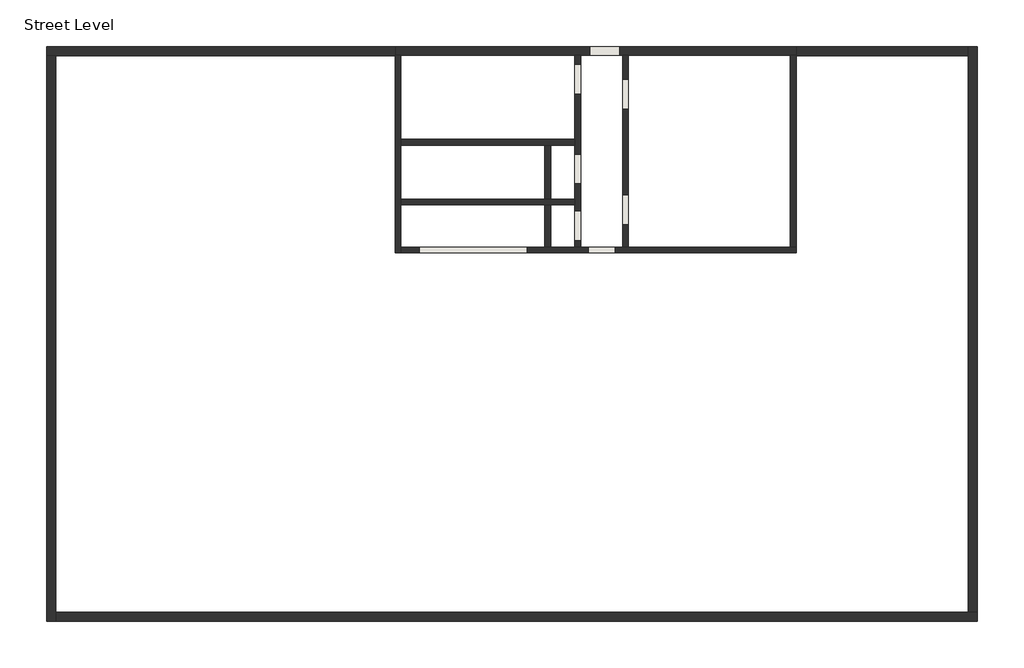
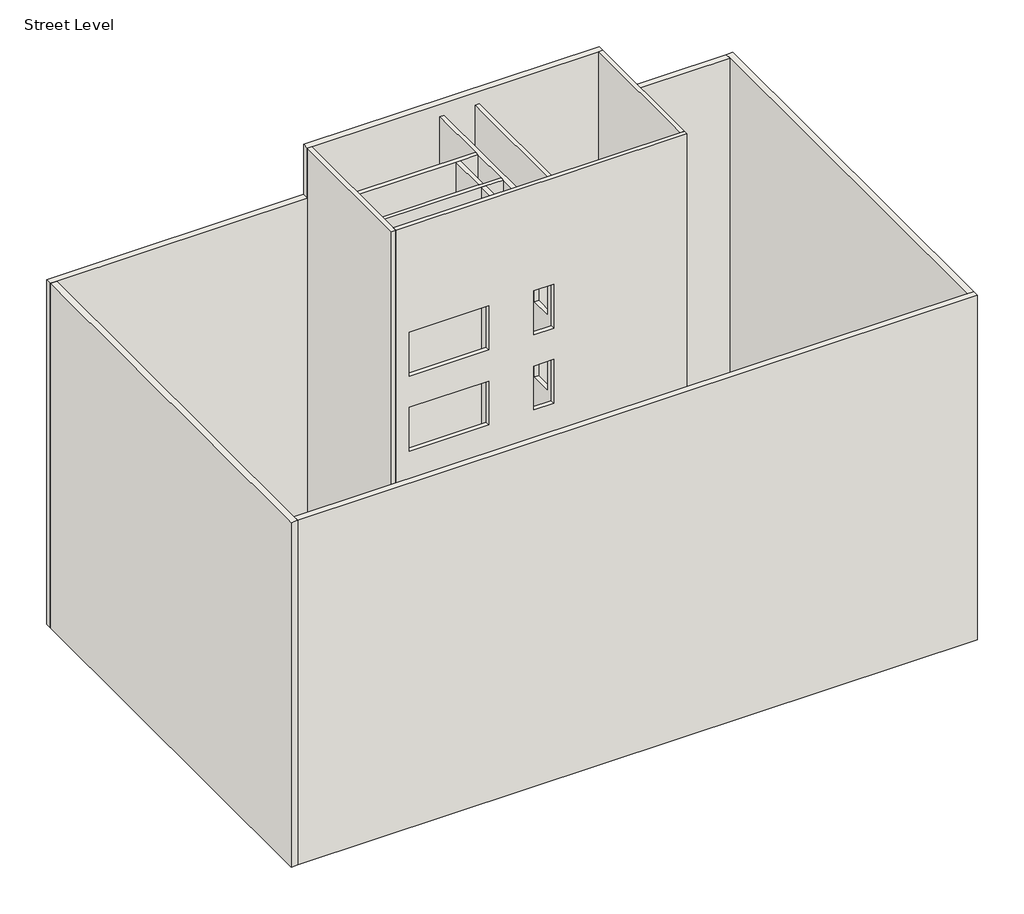
# One storey: 14 walls.
"""IFC4 building model written with IfcOpenShell, lengths in millimetres."""

import ifcopenshell
import ifcopenshell.guid

model = None  # the IFC model being written
_history = None  # IfcOwnerHistory: only IFC2X3 demands one
_inside = {}  # id of a spatial element -> (the spatial element, [elements in it])
_under = {}  # id of a project, library or spatial element -> (it, [spatial elements below it])
_declared = {}  # id of a project -> (the project, [libraries it declares])
_typed = {}  # id of a type object -> (the type object, [elements of that type])
_made_of = {}  # id of a material, layer set ... -> (it, [elements and type objects made of it])


def new_model(schema):
    """Start an empty IFC model of exactly this schema.

    Asked for "IFC4X3", IfcOpenShell would pick the latest addendum, in which some entities
    have other attributes; the version numbers below select the first issue.
    IFC2X3 requires an IfcOwnerHistory on every rooted entity: one is made here for all.
    """
    global model, _history
    if schema == "IFC4X3":
        model = ifcopenshell.file(schema_version=(4, 3, 0, 0))
    else:
        model = ifcopenshell.file(schema=schema)
    _inside.clear()
    _under.clear()
    _declared.clear()
    _typed.clear()
    _made_of.clear()
    _history = None
    if model.schema == "IFC2X3":
        org = make("IfcOrganization", Name="unknown")
        user = make(
            "IfcPersonAndOrganization",
            ThePerson=make("IfcPerson", FamilyName="unknown"),
            TheOrganization=org,
        )
        app = make(
            "IfcApplication",
            ApplicationDeveloper=org,
            Version="unknown",
            ApplicationFullName="unknown",
            ApplicationIdentifier="unknown",
        )
        _history = make(
            "IfcOwnerHistory",
            OwningUser=user,
            OwningApplication=app,
            ChangeAction="ADDED",
            CreationDate=0,
        )
    return model


def make(cls, **values):
    """One entity of the class cls with the attributes given. An attribute that is None is left unset."""
    return model.create_entity(
        cls, **{name: value for name, value in values.items() if value is not None}
    )


def rooted(cls, **values):
    """An entity with a GlobalId (a new one), such as an element, a storey or a relation."""
    return make(cls, GlobalId=ifcopenshell.guid.new(), OwnerHistory=_history, **values)


def si_unit(unit_type, name, prefix=None):
    """IfcSIUnit, for example si_unit("LENGTHUNIT", "METRE", prefix="MILLI")."""
    return make("IfcSIUnit", UnitType=unit_type, Prefix=prefix, Name=name)


def assignment(units):
    """IfcUnitAssignment: the units of a project."""
    return None if units is None else make("IfcUnitAssignment", Units=units)


def point(xyz):
    """IfcCartesianPoint."""
    return None if xyz is None else make("IfcCartesianPoint", Coordinates=xyz)


def direction(xyz):
    """IfcDirection."""
    return None if xyz is None else make("IfcDirection", DirectionRatios=xyz)


def frame(location, z_axis=None, x_axis=None):
    """IfcAxis2Placement3D, a coordinate frame: its origin and axes. An axis left out is left unset."""
    return make(
        "IfcAxis2Placement3D",
        Location=point(location),
        Axis=direction(z_axis),
        RefDirection=direction(x_axis),
    )


def origin():
    """The frame at (0, 0, 0) with its axes left unset."""
    return frame((0.0, 0.0, 0.0))


def place(relative_to, where):
    """IfcLocalPlacement: puts the frame where relative to a parent placement (None: the world)."""
    return make(
        "IfcLocalPlacement", PlacementRelTo=relative_to, RelativePlacement=where
    )


def context(
    kind, dimensions, precision=None, world=None, true_north=None, identifier=None
):
    """IfcGeometricRepresentationContext, for example the 3D "Model" context."""
    return make(
        "IfcGeometricRepresentationContext",
        ContextIdentifier=identifier,
        ContextType=kind,
        CoordinateSpaceDimension=dimensions,
        Precision=precision,
        WorldCoordinateSystem=world,
        TrueNorth=true_north,
    )


def project(units=None, contexts=None):
    """IfcProject with its units and contexts."""
    return rooted(
        "IfcProject",
        Name="project",
        RepresentationContexts=contexts,
        UnitsInContext=assignment(units),
    )


def spatial(cls, under=None, at=None, **own):
    """A site, building, storey or space (cls), placed at a placement, below another one or the project."""
    s = rooted(cls, ObjectPlacement=at, **own)
    if under is not None:
        _under.setdefault(under.id(), (under, []))[1].append(s)
    return s


def polyline(points):
    """IfcPolyline through the points."""
    return make("IfcPolyline", Points=[point(p) for p in points])


def outline(outer, holes=None, kind="AREA"):
    """IfcArbitraryClosedProfileDef: a profile drawn as a closed curve; with holes, ...WithVoids."""
    if holes is None:
        return make("IfcArbitraryClosedProfileDef", ProfileType=kind, OuterCurve=outer)
    return make(
        "IfcArbitraryProfileDefWithVoids",
        ProfileType=kind,
        OuterCurve=outer,
        InnerCurves=holes,
    )


def extrude(swept, where, along, depth):
    """IfcExtrudedAreaSolid: the profile swept, set in the frame where, extruded along a direction by depth."""
    return make(
        "IfcExtrudedAreaSolid",
        SweptArea=swept,
        Position=where,
        ExtrudedDirection=direction(along),
        Depth=depth,
    )


def faces_of(points, faces, orient=None, outer=None):
    """IfcFace entities. A face is a list of loops; a loop is a list of indices into points, from 0.

    orient and outer hold one flag for each loop. By default every Orientation is true, the
    first loop of a face is its IfcFaceOuterBound and the others are IfcFaceBound.
    """
    made = []
    for i, loops in enumerate(faces):
        bounds = []
        for j, loop in enumerate(loops):
            is_outer = j == 0 if outer is None else outer[i][j]
            bounds.append(
                make(
                    "IfcFaceOuterBound" if is_outer else "IfcFaceBound",
                    Bound=make("IfcPolyLoop", Polygon=[points[k] for k in loop]),
                    Orientation=True if orient is None else orient[i][j],
                )
            )
        made.append(make("IfcFace", Bounds=bounds))
    return made


def faceted_brep(points, faces, orient=None, outer=None, voids=None):
    """IfcFacetedBrep: a solid bounded by flat faces; with voids (closed shells), ...WithVoids."""
    shared = [point(p) for p in points]
    hull = make("IfcClosedShell", CfsFaces=faces_of(shared, faces, orient, outer))
    if voids is None:
        return make("IfcFacetedBrep", Outer=hull)
    return make(
        "IfcFacetedBrepWithVoids",
        Outer=hull,
        Voids=[
            make(cls, CfsFaces=faces_of(shared, fs, o, b)) for cls, fs, o, b in voids
        ],
    )


def shape(context_of_items, identifier, shape_type, items):
    """IfcShapeRepresentation: the items that make up one representation, for example the "Body"."""
    return make(
        "IfcShapeRepresentation",
        ContextOfItems=context_of_items,
        RepresentationIdentifier=identifier,
        RepresentationType=shape_type,
        Items=items,
    )


def made_of(thing, what):
    """Note that an element or type object is made of a material, layer set ...; save() writes the relation."""
    if what is not None:
        _made_of.setdefault(what.id(), (what, []))[1].append(thing)
    return thing


def element(
    cls,
    number,
    at=None,
    inside=None,
    cuts=None,
    type_object=None,
    material=None,
    context=None,
    identifier="Body",
    shape_type=None,
    held_by="IfcProductDefinitionShape",
    body=None,
    shapes=None,
    **own,
):
    """One element of the class cls, such as IfcWall. Its Tag is "e" and its number.

    at: its placement. inside: the storey or other place that contains it. cuts: it is an
    opening in that element (IfcRelVoidsElement). A single representation is given by context,
    identifier, shape_type and body (its items); several are given by shapes. held_by: the class
    of the entity that holds the representations. save() writes the other relations.
    """
    e = rooted(cls, Tag="e%d" % number, ObjectPlacement=at, **own)
    if body is not None:
        shapes = [shape(context, identifier, shape_type, body)]
    if shapes is not None:
        e.Representation = make(held_by, Representations=shapes)
    if inside is not None:
        _inside.setdefault(inside.id(), (inside, []))[1].append(e)
    if cuts is not None:
        rooted(
            "IfcRelVoidsElement", RelatingBuildingElement=cuts, RelatedOpeningElement=e
        )
    if type_object is not None:
        _typed.setdefault(type_object.id(), (type_object, []))[1].append(e)
    return made_of(e, material)


def aggregate(whole, parts):
    """IfcRelAggregates: a whole, such as a stair, and the parts it consists of."""
    return rooted("IfcRelAggregates", RelatingObject=whole, RelatedObjects=parts)


def save(model, path):
    """Write the relations noted so far, then the file.

    IfcRelAggregates (storeys below a building ...), IfcRelContainedInSpatialStructure (elements
    in a storey), IfcRelDefinesByType, IfcRelAssociatesMaterial and IfcRelDeclares: one each for
    every whole, place, type object, material and project.
    """
    for whole, parts in _under.values():
        aggregate(whole, parts)
    for where, things in _inside.values():
        rooted(
            "IfcRelContainedInSpatialStructure",
            RelatedElements=things,
            RelatingStructure=where,
        )
    for kind, things in _typed.values():
        rooted("IfcRelDefinesByType", RelatedObjects=things, RelatingType=kind)
    for what, things in _made_of.values():
        rooted("IfcRelAssociatesMaterial", RelatedObjects=things, RelatingMaterial=what)
    for by, libraries in _declared.values():
        rooted("IfcRelDeclares", RelatingContext=by, RelatedDefinitions=libraries)
    model.write(path)


model = new_model("IFC4")

# Units and contexts
model_context = context("Model", 3, world=origin())
ifc_project = project(units=[si_unit("LENGTHUNIT", "METRE", prefix="MILLI")], contexts=[model_context])

# Site, building, storey
site = spatial("IfcSite", under=ifc_project)
building = spatial("IfcBuilding", under=site)
storey = spatial("IfcBuildingStorey", under=building, Name="Street Level", Elevation=-914.4)

# Walls
placement = place(None, origin())
element("IfcWall", 1, ObjectType="Generic - 12\"", at=placement, inside=storey, context=model_context, shape_type="Brep", body=[
    faceted_brep([(-16964.6122732, 9291.5015304, -914.4), (-16659.8122732, 9291.5015304, -914.4), (-5128.2122732, 9291.5015304, -914.4), (-5128.2122732, 9291.5015304, 0.0), (-5128.2122732, 9291.5015304, 3657.6), (-5128.2122732, 9291.5015304, 7315.2), (-5128.2122732, 9291.5015304, 10972.8), (-5128.2122732, 9291.5015304, 14630.4), (-5128.2122732, 9291.5015304, 15849.6), (-16659.8122732, 9291.5015304, 15849.6), (-16964.6122732, 9291.5015304, 15849.6), (-16964.6122732, 9596.3015304, -914.4), (-16964.6122732, 9596.3015304, 15849.6), (-5128.2122732, 9596.3015304, 15849.6), (-5128.2122732, 9596.3015304, -914.4)], [[[0, 1, 2, 3, 4, 5, 6, 7, 8, 9, 10]], [[11, 12, 13, 14]], [[2, 1, 0, 11, 14]], [[10, 9, 8, 13, 12]], [[0, 10, 12, 11]], [[8, 7, 6, 5, 4, 3, 2, 14, 13]]]),
])
element("IfcWall", 2, ObjectType="Generic - 12\"", at=placement, inside=storey, context=model_context, shape_type="Brep", body=[
    faceted_brep([(-16659.8122732, -9910.8984696, -914.4), (-16659.8122732, -9606.0984696, -914.4), (-16659.8122732, 9291.5015304, -914.4), (-16659.8122732, 9291.5015304, 0.0), (-16659.8122732, 9291.5015304, 3657.6), (-16659.8122732, 9291.5015304, 7010.4), (-16659.8122732, 9291.5015304, 7315.2), (-16659.8122732, 9291.5015304, 10972.8), (-16659.8122732, 9291.5015304, 14630.4), (-16659.8122732, 9291.5015304, 15849.6), (-16659.8122732, -9606.0984696, 15849.6), (-16659.8122732, -9910.8984696, 15849.6), (-16964.6122732, -9910.8984696, -914.4), (-16964.6122732, -9910.8984696, 15849.6), (-16964.6122732, 9291.5015304, 15849.6), (-16964.6122732, 9291.5015304, -914.4)], [[[0, 1, 2, 3, 4, 5, 6, 7, 8, 9, 10, 11]], [[12, 13, 14, 15]], [[2, 1, 0, 12, 15]], [[11, 10, 9, 14, 13]], [[0, 11, 13, 12]], [[9, 8, 7, 6, 5, 4, 3, 2, 15, 14]]]),
])
element("IfcWall", 3, ObjectType="Generic - 12\"", at=placement, inside=storey, context=model_context, shape_type="Brep", body=[
    faceted_brep([(14632.9877268, -9606.0984696, -914.4), (14328.1877268, -9606.0984696, -914.4), (-16659.8122732, -9606.0984696, -914.4), (-16659.8122732, -9606.0984696, 0.0), (-16659.8122732, -9606.0984696, 3657.6), (-16659.8122732, -9606.0984696, 7010.4), (-16659.8122732, -9606.0984696, 7315.2), (-16659.8122732, -9606.0984696, 10972.8), (-16659.8122732, -9606.0984696, 14630.4), (-16659.8122732, -9606.0984696, 15849.6), (14328.1877268, -9606.0984696, 15849.6), (14632.9877268, -9606.0984696, 15849.6), (14632.9877268, -9910.8984696, -914.4), (14632.9877268, -9910.8984696, 15849.6), (-16659.8122732, -9910.8984696, 15849.6), (-16659.8122732, -9910.8984696, -914.4)], [[[0, 1, 2, 3, 4, 5, 6, 7, 8, 9, 10, 11]], [[12, 13, 14, 15]], [[2, 1, 0, 12, 15]], [[11, 10, 9, 14, 13]], [[0, 11, 13, 12]], [[9, 8, 7, 6, 5, 4, 3, 2, 15, 14]]]),
])
element("IfcWall", 4, ObjectType="Generic - 12\"", at=placement, inside=storey, context=model_context, shape_type="Brep", body=[
    faceted_brep([(14328.1877268, 9596.3015304, -914.4), (14328.1877268, 9291.5015304, -914.4), (14328.1877268, -9606.0984696, -914.4), (14328.1877268, -9606.0984696, 0.0), (14328.1877268, -9606.0984696, 3657.6), (14328.1877268, -9606.0984696, 7010.4), (14328.1877268, -9606.0984696, 7315.2), (14328.1877268, -9606.0984696, 10972.8), (14328.1877268, -9606.0984696, 14630.4), (14328.1877268, -9606.0984696, 15849.6), (14328.1877268, 9291.5015304, 15849.6), (14328.1877268, 9596.3015304, 15849.6), (14632.9877268, 9596.3015304, -914.4), (14632.9877268, 9596.3015304, 15849.6), (14632.9877268, -9606.0984696, 15849.6), (14632.9877268, -9606.0984696, -914.4)], [[[0, 1, 2, 3, 4, 5, 6, 7, 8, 9, 10, 11]], [[12, 13, 14, 15]], [[2, 1, 0, 12, 15]], [[11, 10, 9, 14, 13]], [[0, 11, 13, 12]], [[9, 8, 7, 6, 5, 4, 3, 2, 15, 14]]]),
])
element("IfcWall", 5, ObjectType="Generic - 12\"", at=placement, inside=storey, context=model_context, shape_type="Brep", body=[
    faceted_brep([(8476.6627268, 9291.5015304, -914.4), (14328.1877268, 9291.5015304, -914.4), (14328.1877268, 9291.5015304, 0.0), (14328.1877268, 9291.5015304, 3352.8), (14328.1877268, 9291.5015304, 3657.6), (14328.1877268, 9291.5015304, 7010.4), (14328.1877268, 9291.5015304, 7315.2), (14328.1877268, 9291.5015304, 10668.0), (14328.1877268, 9291.5015304, 10972.8), (14328.1877268, 9291.5015304, 14630.4), (14328.1877268, 9291.5015304, 15849.6), (8476.6627268, 9291.5015304, 15849.6), (8476.6627268, 9596.3015304, -914.4), (8476.6627268, 9596.3015304, 15849.6), (14328.1877268, 9596.3015304, 15849.6), (14328.1877268, 9596.3015304, -914.4)], [[[0, 1, 2, 3, 4, 5, 6, 7, 8, 9, 10, 11]], [[12, 13, 14, 15]], [[1, 0, 12, 15]], [[11, 10, 14, 13]], [[10, 9, 8, 7, 6, 5, 4, 3, 2, 1, 15, 14]], [[0, 11, 13, 12]]]),
])
element("IfcWall", 6, ObjectType="Generic - 12\" Masonry", at=placement, inside=storey, context=model_context, shape_type="Brep", body=[
    faceted_brep([(-5128.2122732, 9301.0265304, 18288.0), (-5128.2122732, 9301.0265304, -914.4), (-4934.5372732, 9301.0265304, -914.4), (967.7877268, 9301.0265304, -914.4), (1161.4627268, 9301.0265304, -914.4), (2593.3877268, 9301.0265304, -914.4), (2787.0627268, 9301.0265304, -914.4), (8282.9877268, 9301.0265304, -914.4), (8476.6627268, 9301.0265304, -914.4), (8476.6627268, 9301.0265304, 18288.0), (8282.9877268, 9301.0265304, 18288.0), (-4934.5372732, 9301.0265304, 18288.0), (2491.7877268, 9301.0265304, 0.0), (1475.7877268, 9301.0265304, 0.0), (1475.7877268, 9301.0265304, 2235.2), (2491.7877268, 9301.0265304, 2235.2), (-5128.2122732, 9596.3015304, -914.4), (-5128.2122732, 9596.3015304, 18288.0), (8476.6627268, 9596.3015304, 18288.0), (8476.6627268, 9596.3015304, -914.4), (2491.7877268, 9596.3015304, 0.0), (2491.7877268, 9596.3015304, 2235.2), (1475.7877268, 9596.3015304, 2235.2), (1475.7877268, 9596.3015304, 0.0)], [[[0, 1, 2, 3, 4, 5, 6, 7, 8, 9, 10, 11], [12, 13, 14, 15]], [[16, 17, 18, 19], [20, 21, 22, 23]], [[8, 7, 6, 5, 4, 3, 2, 1, 16, 19]], [[0, 11, 10, 9, 18, 17]], [[20, 23, 13, 12]], [[23, 22, 14, 13]], [[22, 21, 15, 14]], [[21, 20, 12, 15]], [[0, 17, 16, 1]], [[8, 19, 18, 9]]]),
])
element("IfcWall", 7, ObjectType="Generic - 8\" Masonry", at=placement, inside=storey, context=model_context, shape_type="Brep", body=[
    faceted_brep([(-5128.2122732, 9301.0265304, 18288.0), (-5128.2122732, 9301.0265304, -914.4), (-5128.2122732, 2595.4265304, -914.4), (-5128.2122732, 2595.4265304, 18288.0), (-4934.5372732, 9301.0265304, -914.4), (-4934.5372732, 9301.0265304, 18288.0), (-4934.5372732, 2789.1015304, 18288.0), (-4934.5372732, 2595.4265304, 18288.0), (-4934.5372732, 2595.4265304, -914.4), (-4934.5372732, 2789.1015304, -914.4), (-4934.5372732, 4221.0265304, -914.4), (-4934.5372732, 4414.7015304, -914.4), (-4934.5372732, 6253.0265304, -914.4), (-4934.5372732, 6446.7015304, -914.4)], [[[0, 1, 2, 3]], [[4, 5, 6, 7, 8, 9, 10, 11, 12, 13]], [[2, 1, 4, 13, 12, 11, 10, 9, 8]], [[0, 3, 7, 6, 5]], [[3, 2, 8, 7]], [[0, 5, 4, 1]]]),
])
element("IfcWall", 8, ObjectType="Generic - 8\" Masonry", at=placement, inside=storey, context=model_context, shape_type="Brep", body=[
    faceted_brep([(8476.6627268, 2789.1015304, -914.4), (8282.9877268, 2789.1015304, -914.4), (2787.0627268, 2789.1015304, -914.4), (2593.3877268, 2789.1015304, -914.4), (1161.4627268, 2789.1015304, -914.4), (967.7877268, 2789.1015304, -914.4), (145.4627268, 2789.1015304, -914.4), (-48.2122732, 2789.1015304, -914.4), (-4934.5372732, 2789.1015304, -914.4), (-4934.5372732, 2789.1015304, 18288.0), (8282.9877268, 2789.1015304, 18288.0), (8476.6627268, 2789.1015304, 18288.0), (-653.0497732, 2789.1015304, 2133.6), (-4310.6497732, 2789.1015304, 2133.6), (-4310.6497732, 2789.1015304, 0.0), (-653.0497732, 2789.1015304, 0.0), (2344.1502268, 2789.1015304, 2133.6), (1429.7502268, 2789.1015304, 2133.6), (1429.7502268, 2789.1015304, 0.0), (2344.1502268, 2789.1015304, 0.0), (2344.1502268, 2789.1015304, 5791.2), (1429.7502268, 2789.1015304, 5791.2), (1429.7502268, 2789.1015304, 3657.6), (2344.1502268, 2789.1015304, 3657.6), (-653.0497732, 2789.1015304, 5791.2), (-4310.6497732, 2789.1015304, 5791.2), (-4310.6497732, 2789.1015304, 3657.6), (-653.0497732, 2789.1015304, 3657.6), (2344.1502268, 2789.1015304, 9448.8), (1429.7502268, 2789.1015304, 9448.8), (1429.7502268, 2789.1015304, 7315.2), (2344.1502268, 2789.1015304, 7315.2), (-653.0497732, 2789.1015304, 9448.8), (-4310.6497732, 2789.1015304, 9448.8), (-4310.6497732, 2789.1015304, 7315.2), (-653.0497732, 2789.1015304, 7315.2), (2344.1502268, 2789.1015304, 13106.4), (1429.7502268, 2789.1015304, 13106.4), (1429.7502268, 2789.1015304, 10972.8), (2344.1502268, 2789.1015304, 10972.8), (-653.0497732, 2789.1015304, 13106.4), (-4310.6497732, 2789.1015304, 13106.4), (-4310.6497732, 2789.1015304, 10972.8), (-653.0497732, 2789.1015304, 10972.8), (8476.6627268, 2595.4265304, -914.4), (8476.6627268, 2595.4265304, 18288.0), (-4934.5372732, 2595.4265304, 18288.0), (-4934.5372732, 2595.4265304, -914.4), (-653.0497732, 2595.4265304, 2133.6), (-653.0497732, 2595.4265304, 0.0), (-4310.6497732, 2595.4265304, 0.0), (-4310.6497732, 2595.4265304, 2133.6), (2344.1502268, 2595.4265304, 2133.6), (2344.1502268, 2595.4265304, 0.0), (1429.7502268, 2595.4265304, 0.0), (1429.7502268, 2595.4265304, 2133.6), (2344.1502268, 2595.4265304, 5791.2), (2344.1502268, 2595.4265304, 3657.6), (1429.7502268, 2595.4265304, 3657.6), (1429.7502268, 2595.4265304, 5791.2), (-653.0497732, 2595.4265304, 5791.2), (-653.0497732, 2595.4265304, 3657.6), (-4310.6497732, 2595.4265304, 3657.6), (-4310.6497732, 2595.4265304, 5791.2), (2344.1502268, 2595.4265304, 9448.8), (2344.1502268, 2595.4265304, 7315.2), (1429.7502268, 2595.4265304, 7315.2), (1429.7502268, 2595.4265304, 9448.8), (-653.0497732, 2595.4265304, 9448.8), (-653.0497732, 2595.4265304, 7315.2), (-4310.6497732, 2595.4265304, 7315.2), (-4310.6497732, 2595.4265304, 9448.8), (2344.1502268, 2595.4265304, 13106.4), (2344.1502268, 2595.4265304, 10972.8), (1429.7502268, 2595.4265304, 10972.8), (1429.7502268, 2595.4265304, 13106.4), (-653.0497732, 2595.4265304, 13106.4), (-653.0497732, 2595.4265304, 10972.8), (-4310.6497732, 2595.4265304, 10972.8), (-4310.6497732, 2595.4265304, 13106.4)], [[[0, 1, 2, 3, 4, 5, 6, 7, 8, 9, 10, 11], [12, 13, 14, 15], [16, 17, 18, 19], [20, 21, 22, 23], [24, 25, 26, 27], [28, 29, 30, 31], [32, 33, 34, 35], [36, 37, 38, 39], [40, 41, 42, 43]], [[44, 45, 46, 47], [48, 49, 50, 51], [52, 53, 54, 55], [56, 57, 58, 59], [60, 61, 62, 63], [64, 65, 66, 67], [68, 69, 70, 71], [72, 73, 74, 75], [76, 77, 78, 79]], [[8, 7, 6, 5, 4, 3, 2, 1, 0, 44, 47]], [[11, 10, 9, 46, 45]], [[9, 8, 47, 46]], [[0, 11, 45, 44]], [[49, 48, 12, 15]], [[50, 49, 15, 14]], [[51, 50, 14, 13]], [[48, 51, 13, 12]], [[53, 52, 16, 19]], [[54, 53, 19, 18]], [[55, 54, 18, 17]], [[52, 55, 17, 16]], [[57, 56, 20, 23]], [[58, 57, 23, 22]], [[59, 58, 22, 21]], [[56, 59, 21, 20]], [[61, 60, 24, 27]], [[62, 61, 27, 26]], [[63, 62, 26, 25]], [[60, 63, 25, 24]], [[65, 64, 28, 31]], [[66, 65, 31, 30]], [[67, 66, 30, 29]], [[64, 67, 29, 28]], [[69, 68, 32, 35]], [[70, 69, 35, 34]], [[71, 70, 34, 33]], [[68, 71, 33, 32]], [[73, 72, 36, 39]], [[74, 73, 39, 38]], [[75, 74, 38, 37]], [[72, 75, 37, 36]], [[77, 76, 40, 43]], [[78, 77, 43, 42]], [[79, 78, 42, 41]], [[76, 79, 41, 40]]]),
])
element("IfcWall", 9, ObjectType="Generic - 8\" Masonry", at=placement, inside=storey, context=model_context, shape_type="SweptSolid", body=[
    extrude(outline(polyline([(8282.9877268, 2789.1015304), (8282.9877268, 9301.0265304), (8476.6627268, 9301.0265304), (8476.6627268, 2789.1015304), (8282.9877268, 2789.1015304)])), frame((0.0, 0.0, -914.4), z_axis=(0.0, 0.0, 1.0), x_axis=(1.0, 0.0, 0.0)), (0.0, 0.0, 1.0), 19202.4),
])
element("IfcWall", 10, ObjectType="Generic - 8\" Masonry", at=placement, inside=storey, context=model_context, shape_type="Brep", body=[
    faceted_brep([(1161.4627268, 2789.1015304, -914.4), (1161.4627268, 9301.0265304, -914.4), (1161.4627268, 9301.0265304, 17678.4), (1161.4627268, 2789.1015304, 17678.4), (1161.4627268, 8996.2265304, 0.0), (1161.4627268, 7980.2265304, 0.0), (1161.4627268, 7980.2265304, 2235.2), (1161.4627268, 8996.2265304, 2235.2), (1161.4627268, 5948.2265304, 0.0), (1161.4627268, 4932.2265304, 0.0), (1161.4627268, 4932.2265304, 2235.2), (1161.4627268, 5948.2265304, 2235.2), (1161.4627268, 4017.8265304, 0.0), (1161.4627268, 3001.8265304, 0.0), (1161.4627268, 3001.8265304, 2235.2), (1161.4627268, 4017.8265304, 2235.2), (1161.4627268, 4017.8265304, 3657.6), (1161.4627268, 3001.8265304, 3657.6), (1161.4627268, 3001.8265304, 5892.8), (1161.4627268, 4017.8265304, 5892.8), (1161.4627268, 5948.2265304, 3657.6), (1161.4627268, 4932.2265304, 3657.6), (1161.4627268, 4932.2265304, 5892.8), (1161.4627268, 5948.2265304, 5892.8), (1161.4627268, 8996.2265304, 3657.6), (1161.4627268, 7980.2265304, 3657.6), (1161.4627268, 7980.2265304, 5892.8), (1161.4627268, 8996.2265304, 5892.8), (1161.4627268, 4017.8265304, 7315.2), (1161.4627268, 3001.8265304, 7315.2), (1161.4627268, 3001.8265304, 9550.4), (1161.4627268, 4017.8265304, 9550.4), (1161.4627268, 5948.2265304, 7315.2), (1161.4627268, 4932.2265304, 7315.2), (1161.4627268, 4932.2265304, 9550.4), (1161.4627268, 5948.2265304, 9550.4), (1161.4627268, 8996.2265304, 7315.2), (1161.4627268, 7980.2265304, 7315.2), (1161.4627268, 7980.2265304, 9550.4), (1161.4627268, 8996.2265304, 9550.4), (1161.4627268, 4017.8265304, 10972.8), (1161.4627268, 3001.8265304, 10972.8), (1161.4627268, 3001.8265304, 13208.0), (1161.4627268, 4017.8265304, 13208.0), (1161.4627268, 5948.2265304, 10972.8), (1161.4627268, 4932.2265304, 10972.8), (1161.4627268, 4932.2265304, 13208.0), (1161.4627268, 5948.2265304, 13208.0), (1161.4627268, 8996.2265304, 10972.8), (1161.4627268, 7980.2265304, 10972.8), (1161.4627268, 7980.2265304, 13208.0), (1161.4627268, 8996.2265304, 13208.0), (967.7877268, 2789.1015304, -914.4), (967.7877268, 2789.1015304, 17678.4), (967.7877268, 4221.0265304, 17678.4), (967.7877268, 4414.7015304, 17678.4), (967.7877268, 6253.0265304, 17678.4), (967.7877268, 6446.7015304, 17678.4), (967.7877268, 9301.0265304, 17678.4), (967.7877268, 9301.0265304, -914.4), (967.7877268, 6446.7015304, -914.4), (967.7877268, 6253.0265304, -914.4), (967.7877268, 4414.7015304, -914.4), (967.7877268, 4221.0265304, -914.4), (967.7877268, 8996.2265304, 0.0), (967.7877268, 8996.2265304, 2235.2), (967.7877268, 7980.2265304, 2235.2), (967.7877268, 7980.2265304, 0.0), (967.7877268, 5948.2265304, 0.0), (967.7877268, 5948.2265304, 2235.2), (967.7877268, 4932.2265304, 2235.2), (967.7877268, 4932.2265304, 0.0), (967.7877268, 4017.8265304, 0.0), (967.7877268, 4017.8265304, 2235.2), (967.7877268, 3001.8265304, 2235.2), (967.7877268, 3001.8265304, 0.0), (967.7877268, 4017.8265304, 3657.6), (967.7877268, 4017.8265304, 5892.8), (967.7877268, 3001.8265304, 5892.8), (967.7877268, 3001.8265304, 3657.6), (967.7877268, 5948.2265304, 3657.6), (967.7877268, 5948.2265304, 5892.8), (967.7877268, 4932.2265304, 5892.8), (967.7877268, 4932.2265304, 3657.6), (967.7877268, 8996.2265304, 3657.6), (967.7877268, 8996.2265304, 5892.8), (967.7877268, 7980.2265304, 5892.8), (967.7877268, 7980.2265304, 3657.6), (967.7877268, 4017.8265304, 7315.2), (967.7877268, 4017.8265304, 9550.4), (967.7877268, 3001.8265304, 9550.4), (967.7877268, 3001.8265304, 7315.2), (967.7877268, 5948.2265304, 7315.2), (967.7877268, 5948.2265304, 9550.4), (967.7877268, 4932.2265304, 9550.4), (967.7877268, 4932.2265304, 7315.2), (967.7877268, 8996.2265304, 7315.2), (967.7877268, 8996.2265304, 9550.4), (967.7877268, 7980.2265304, 9550.4), (967.7877268, 7980.2265304, 7315.2), (967.7877268, 4017.8265304, 10972.8), (967.7877268, 4017.8265304, 13208.0), (967.7877268, 3001.8265304, 13208.0), (967.7877268, 3001.8265304, 10972.8), (967.7877268, 5948.2265304, 10972.8), (967.7877268, 5948.2265304, 13208.0), (967.7877268, 4932.2265304, 13208.0), (967.7877268, 4932.2265304, 10972.8), (967.7877268, 8996.2265304, 10972.8), (967.7877268, 8996.2265304, 13208.0), (967.7877268, 7980.2265304, 13208.0), (967.7877268, 7980.2265304, 10972.8)], [[[0, 1, 2, 3], [4, 5, 6, 7], [8, 9, 10, 11], [12, 13, 14, 15], [16, 17, 18, 19], [20, 21, 22, 23], [24, 25, 26, 27], [28, 29, 30, 31], [32, 33, 34, 35], [36, 37, 38, 39], [40, 41, 42, 43], [44, 45, 46, 47], [48, 49, 50, 51]], [[52, 53, 54, 55, 56, 57, 58, 59, 60, 61, 62, 63], [64, 65, 66, 67], [68, 69, 70, 71], [72, 73, 74, 75], [76, 77, 78, 79], [80, 81, 82, 83], [84, 85, 86, 87], [88, 89, 90, 91], [92, 93, 94, 95], [96, 97, 98, 99], [100, 101, 102, 103], [104, 105, 106, 107], [108, 109, 110, 111]], [[1, 0, 52, 63, 62, 61, 60, 59]], [[3, 2, 58, 57, 56, 55, 54, 53]], [[65, 64, 4, 7]], [[66, 65, 7, 6]], [[67, 66, 6, 5]], [[64, 67, 5, 4]], [[69, 68, 8, 11]], [[70, 69, 11, 10]], [[71, 70, 10, 9]], [[68, 71, 9, 8]], [[73, 72, 12, 15]], [[74, 73, 15, 14]], [[75, 74, 14, 13]], [[72, 75, 13, 12]], [[0, 3, 53, 52]], [[2, 1, 59, 58]], [[77, 76, 16, 19]], [[78, 77, 19, 18]], [[79, 78, 18, 17]], [[76, 79, 17, 16]], [[81, 80, 20, 23]], [[82, 81, 23, 22]], [[83, 82, 22, 21]], [[80, 83, 21, 20]], [[85, 84, 24, 27]], [[86, 85, 27, 26]], [[87, 86, 26, 25]], [[84, 87, 25, 24]], [[89, 88, 28, 31]], [[90, 89, 31, 30]], [[91, 90, 30, 29]], [[88, 91, 29, 28]], [[93, 92, 32, 35]], [[94, 93, 35, 34]], [[95, 94, 34, 33]], [[92, 95, 33, 32]], [[97, 96, 36, 39]], [[98, 97, 39, 38]], [[99, 98, 38, 37]], [[96, 99, 37, 36]], [[101, 100, 40, 43]], [[102, 101, 43, 42]], [[103, 102, 42, 41]], [[100, 103, 41, 40]], [[105, 104, 44, 47]], [[106, 105, 47, 46]], [[107, 106, 46, 45]], [[104, 107, 45, 44]], [[109, 108, 48, 51]], [[110, 109, 51, 50]], [[111, 110, 50, 49]], [[108, 111, 49, 48]]]),
])
element("IfcWall", 11, ObjectType="Generic - 8\" Masonry", at=placement, inside=storey, context=model_context, shape_type="SweptSolid", body=[
    extrude(outline(polyline([(9301.0265304, -914.4), (2789.1015304, -914.4), (2789.1015304, 17678.4), (9301.0265304, 17678.4), (9301.0265304, -914.4)]), holes=[polyline([(3551.1015304, 0.0), (4567.1015304, 0.0), (4567.1015304, 2235.2), (3551.1015304, 2235.2), (3551.1015304, 0.0)]), polyline([(8488.2265304, 0.0), (8488.2265304, 2235.2), (7472.2265304, 2235.2), (7472.2265304, 0.0), (8488.2265304, 0.0)]), polyline([(8488.2265304, 3657.6), (8488.2265304, 5892.8), (7472.2265304, 5892.8), (7472.2265304, 3657.6), (8488.2265304, 3657.6)]), polyline([(3551.1015304, 3657.6), (4567.1015304, 3657.6), (4567.1015304, 5892.8), (3551.1015304, 5892.8), (3551.1015304, 3657.6)]), polyline([(8488.2265304, 7315.2), (8488.2265304, 9550.4), (7472.2265304, 9550.4), (7472.2265304, 7315.2), (8488.2265304, 7315.2)]), polyline([(3551.1015304, 7315.2), (4567.1015304, 7315.2), (4567.1015304, 9550.4), (3551.1015304, 9550.4), (3551.1015304, 7315.2)]), polyline([(8488.2265304, 10972.8), (8488.2265304, 13208.0), (7472.2265304, 13208.0), (7472.2265304, 10972.8), (8488.2265304, 10972.8)]), polyline([(3551.1015304, 10972.8), (4567.1015304, 10972.8), (4567.1015304, 13208.0), (3551.1015304, 13208.0), (3551.1015304, 10972.8)])]), frame((2593.3877268, 0.0, 0.0), z_axis=(1.0, 0.0, 0.0), x_axis=(0.0, 1.0, 0.0)), (0.0, 0.0, 1.0), 193.675),
])
element("IfcWall", 12, ObjectType="Generic - 8\" Masonry", at=placement, inside=storey, context=model_context, shape_type="Brep", body=[
    faceted_brep([(967.7877268, 6446.7015304, -914.4), (-4934.5372732, 6446.7015304, -914.4), (-4934.5372732, 6446.7015304, 17678.4), (967.7877268, 6446.7015304, 17678.4), (967.7877268, 6253.0265304, -914.4), (967.7877268, 6253.0265304, 17678.4), (145.4627268, 6253.0265304, 17678.4), (-48.2122732, 6253.0265304, 17678.4), (-4934.5372732, 6253.0265304, 17678.4), (-4934.5372732, 6253.0265304, -914.4), (-48.2122732, 6253.0265304, -914.4), (145.4627268, 6253.0265304, -914.4)], [[[0, 1, 2, 3]], [[4, 5, 6, 7, 8, 9, 10, 11]], [[1, 0, 4, 11, 10, 9]], [[3, 2, 8, 7, 6, 5]], [[0, 3, 5, 4]], [[2, 1, 9, 8]]]),
])
element("IfcWall", 13, ObjectType="Generic - 8\" Masonry", at=placement, inside=storey, context=model_context, shape_type="Brep", body=[
    faceted_brep([(-4934.5372732, 4221.0265304, -914.4), (-48.2122732, 4221.0265304, -914.4), (145.4627268, 4221.0265304, -914.4), (967.7877268, 4221.0265304, -914.4), (967.7877268, 4221.0265304, 17678.4), (145.4627268, 4221.0265304, 17678.4), (-48.2122732, 4221.0265304, 17678.4), (-4934.5372732, 4221.0265304, 17678.4), (-4934.5372732, 4414.7015304, -914.4), (-4934.5372732, 4414.7015304, 17678.4), (-48.2122732, 4414.7015304, 17678.4), (145.4627268, 4414.7015304, 17678.4), (967.7877268, 4414.7015304, 17678.4), (967.7877268, 4414.7015304, -914.4), (145.4627268, 4414.7015304, -914.4), (-48.2122732, 4414.7015304, -914.4)], [[[0, 1, 2, 3, 4, 5, 6, 7]], [[8, 9, 10, 11, 12, 13, 14, 15]], [[3, 2, 1, 0, 8, 15, 14, 13]], [[7, 6, 5, 4, 12, 11, 10, 9]], [[4, 3, 13, 12]], [[0, 7, 9, 8]]]),
])
element("IfcWall", 14, ObjectType="Generic - 8\" Masonry", at=placement, inside=storey, context=model_context, shape_type="SweptSolid", body=[
    extrude(outline(polyline([(-48.2122732, 6253.0265304), (145.4627268, 6253.0265304), (145.4627268, 4414.7015304), (-48.2122732, 4414.7015304), (-48.2122732, 6253.0265304)])), frame((0.0, 0.0, -914.4), z_axis=(0.0, 0.0, 1.0), x_axis=(1.0, 0.0, 0.0)), (0.0, 0.0, 1.0), 18592.8),
    extrude(outline(polyline([(145.4627268, 2789.1015304), (-48.2122732, 2789.1015304), (-48.2122732, 4221.0265304), (145.4627268, 4221.0265304), (145.4627268, 2789.1015304)])), frame((0.0, 0.0, -914.4), z_axis=(0.0, 0.0, 1.0), x_axis=(1.0, 0.0, 0.0)), (0.0, 0.0, 1.0), 18592.8),
])

save(model, "model.ifc")

# Revit data of these elements
# Project information
#   Organization Name = "G3B Press"
#   Organization Description = "Paul F. Aubin Cosulting Services, Inc."
#   Building Name = "Revit Essentials for Architecture"
#   Author = "Paul F. Aubin"
#   Author Website = "https://www.paulaubin.com"
#   Copyright = "Copyright © 2020 Paul F Aubin, all rights reserved"
#   Project Issue Date = "8/1/2020"
#   Project Status = "Design Development"
#   Client Name = "Vertical Circulation"
#   Project Address = "123 State ST\nSuite 301\nChicago, IL 60606"
#   Project Name = "08 Commercial"
#   Project Number = "2020.04A"
# Grids (mm)
#   "1": line (-22547.601, -9504.498) -> (19277.595, -9504.498)
#   "2": line (-22547.601, -3408.498) -> (19277.595, -3408.498)
#   "3": line (-22547.601, 3093.902) -> (19277.595, 3093.902)
#   "4": line (-22547.601, 9189.902) -> (19277.595, 9189.902)
#   "A": line (-16558.212, 12259.726) -> (-16558.212, -14197.104)
#   "B": line (-9801.812, 12259.726) -> (-9801.812, -14197.104)
#   "C": line (-5433.012, 12259.726) -> (-5433.012, -14197.104)
#   "D": line (3101.388, 12259.726) -> (3101.388, -14197.104)
#   "E": line (7470.188, 12259.726) -> (7470.188, -14197.104)
#   "F": line (14226.588, 12259.726) -> (14226.588, -14197.104)
#   "C.3": line (-2689.812, -15151.11) -> (-2689.812, -5965.346)
#   "C.7": line (358.188, -15151.11) -> (358.188, -5965.346)
# Type "Generic - 12\""
#   Assembly Code = "B2010"
#   Layers, outside or top first: 1' - 0" no material (function 1)
# Type "Generic - 12\" Masonry"
#   Assembly Code = "B2010"
#   Layers, outside or top first: 0' - 11 5/8" "Concrete Masonry Units" (function 1)
# Type "Generic - 8\" Masonry"
#   Assembly Code = "B2010"
#   Layers, outside or top first: 0' - 7 5/8" "Concrete Masonry Units" (function 1)
# Elements 1, 2, 3, 4, 5 (IfcWall, "Generic - 12\"")
#   Top Offset = 4' - 0"
#   Base Offset = 0' - 0"
#   wall height = 55' - 0"
#   Phase Created = New Construction
#   Base Constraint = Street Level
#   Top Constraint = Roof
#   Materials on its faces: "Default Wall"
# Element 6 (IfcWall, "Generic - 12\" Masonry")
#   Top Offset = 12' - 0"
#   Base Offset = 0' - 0"
#   wall height = 63' - 0"
#   Phase Created = New Construction
#   Base Constraint = Street Level
#   Top Constraint = Roof
#   Materials on its faces: "Concrete Masonry Units"
# Elements 7, 8, 9 (IfcWall, "Generic - 8\" Masonry")
#   Comments = ""
#   Top Offset = 12' - 0"
#   Base Offset = 0' - 0"
#   wall height = 63' - 0"
#   Phase Created = New Construction
#   Base Constraint = Street Level
#   Top Constraint = Roof
#   Materials on its faces: "Concrete Masonry Units"
# Elements 10, 11, 12, 13, 14 (IfcWall, "Generic - 8\" Masonry")
#   Top Offset = 10' - 0"
#   Base Offset = 0' - 0"
#   wall height = 61' - 0"
#   Phase Created = New Construction
#   Base Constraint = Street Level
#   Top Constraint = Roof
#   Materials on its faces: "Concrete Masonry Units"
# Materials
#   "Concrete Masonry Units": class "Masonry", colour RGB 227 227 227, transparency 0, Description = "Concrete masonry units", Cost = 0
#   "Default Wall": class "Miscellaneous", colour RGB 128 128 128, transparency 0, Cost = 0
